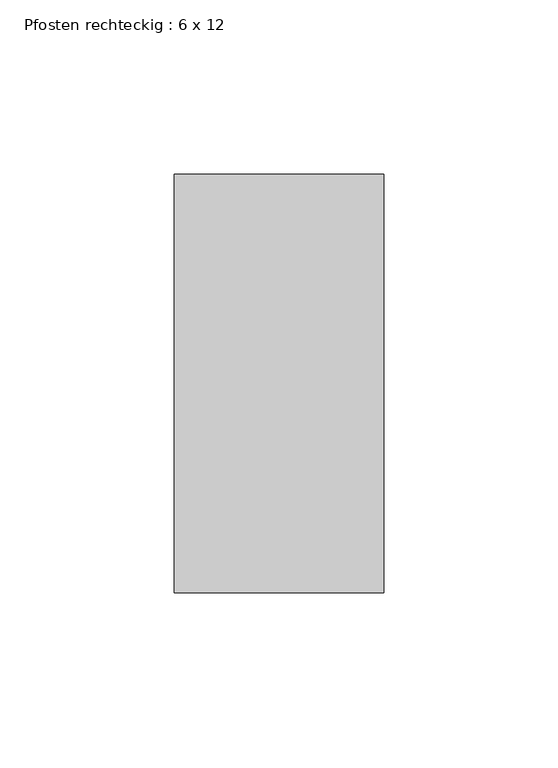
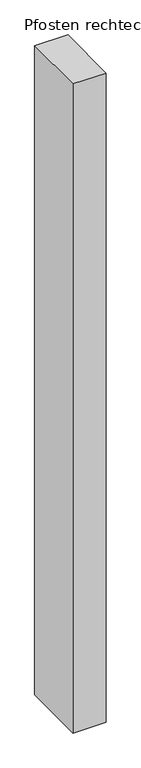
"""IFC4 building model written with IfcOpenShell, lengths in millimetres: member geometry, Pfosten rechteckig : 6 x 12."""

from ifc_helpers import new_model, si_unit, frame, origin, place, context, project, spatial, polyline, outline, extrude, source, transform, mapped, element, save


def pfosten_rechteckig_6_x_12_f8cf5b5c(model_context):
    return source(origin(), model_context, "Body", "SweptSolid", [
        extrude(outline(polyline([(0.0, 60.0), (0.0, -60.0), (-60.0, -60.0), (-60.0, 60.0), (0.0, 60.0)])), frame((0.0, 0.0, -1240.0), z_axis=(0.0, 0.0, 1.0), x_axis=(1.0, 0.0, 0.0)), (0.0, 0.0, 1.0), 1240.0),
    ])


if __name__ == "__main__":
    model = new_model("IFC4")
    model_context = context("Model", 3, world=origin())
    ifc_project = project(units=[si_unit("LENGTHUNIT", "METRE", prefix="MILLI")], contexts=[model_context])
    site = spatial("IfcSite", under=ifc_project)
    building = spatial("IfcBuilding", under=site)
    placement = place(None, origin())
    pfosten_rechteckig_6_x_12_shape = pfosten_rechteckig_6_x_12_f8cf5b5c(model_context)
    element("IfcMember", 1, ObjectType="Pfosten rechteckig : 6 x 12", at=placement, inside=building, context=model_context, shape_type="MappedRepresentation", body=[
        mapped(pfosten_rechteckig_6_x_12_shape, transform((0.0, 0.0, 0.0), x_axis=(1.0, 0.0, 0.0), y_axis=(0.0, 1.0, 0.0), z_axis=(0.0, 0.0, 1.0))),
    ])
    save(model, "model.ifc")

# Revit data of these elements
# Type "Pfosten rechteckig : 6 x 12"
#   built-in parameter 1007304 = 0.393701 (stored number, unit not read)
#   built-in parameter 1007301 = 0.0984252 (stored number, unit not read)
#   built-in parameter 1007300 = 0.0984252 (stored number, unit not read)
# Element 1 (IfcMember, "Pfosten rechteckig : 6 x 12")
#   Materials on its faces: "Metall - verzinkt"
# Materials
#   "Metall - verzinkt": class "Allgemeines", colour RGB 200 200 200, transparency 0, Cost = 0
